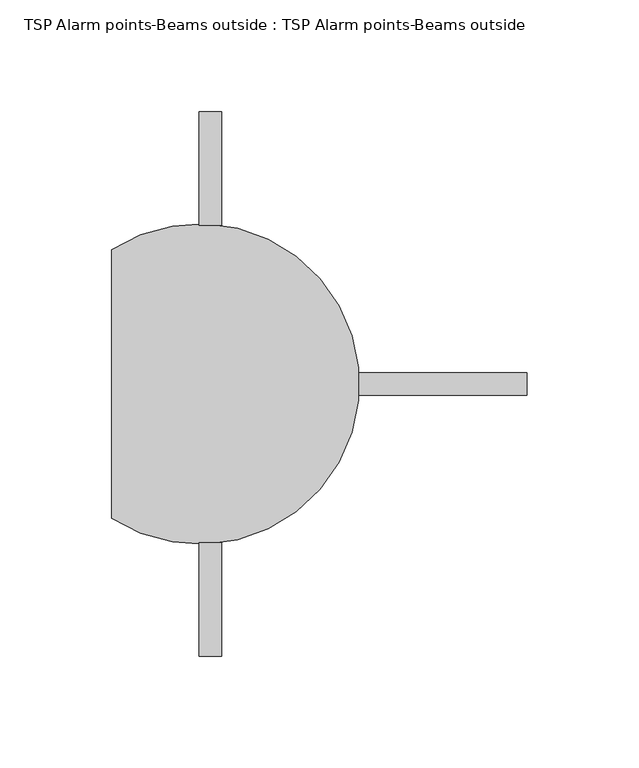
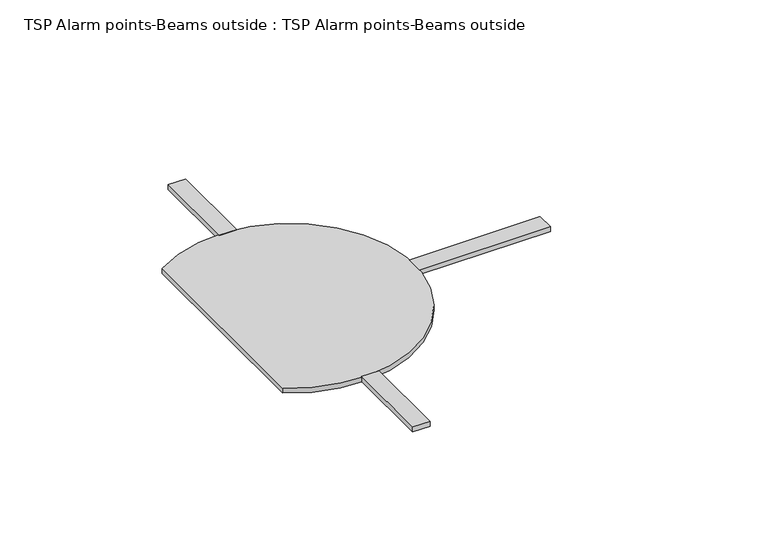
"""IFC4 building model written with IfcOpenShell, lengths in millimetres: proxy geometry, TSP Alarm points-Beams outside : TSP Alarm points-Beams outside."""

from ifc_helpers import new_model, si_unit, point, frame_2d, origin, origin_with_axes, place, context, project, spatial, polyline, circle_curve, trimmed, segment, composite_curve, outline, extrude, source, transform, mapped, element, save


def tsp_alarm_points_beams_outside_tsp_alarm_points_beams_36a8186e(model_context):
    return source(origin(), model_context, "Body", "SweptSolid", [
        extrude(outline(polyline([(75.7016567, 5.0), (75.7016567, -5.0), (0.5268886, -5.0), (0.5268886, 5.0), (75.7016567, 5.0)])), origin_with_axes(), (0.0, 0.0, 1.0), 3.0),
        extrude(outline(polyline([(-70.9090909, 121.6107476), (-60.9090909, 121.6107476), (-60.9090909, 70.9090909), (-70.9090909, 70.9090909), (-70.9090909, 121.6107476)])), origin_with_axes(), (0.0, 0.0, 1.0), 3.0),
        extrude(outline(polyline([(-70.9090909, -121.6107476), (-70.9090909, -70.9090909), (-60.9090909, -70.9090909), (-60.9090909, -121.6107476), (-70.9090909, -121.6107476)])), origin_with_axes(), (0.0, 0.0, 1.0), 3.0),
        extrude(outline(composite_curve([segment(trimmed(circle_curve(frame_2d((-70.9090909, 0.0)), 71.6107476), [point((-110.0, 60.0))], [point((-110.0, -60.0))], False, "CARTESIAN"), True, "CONTINUOUS"), segment(polyline([(-110.0, -60.0), (-110.0, 60.0)]), True, "CONTINUOUS")], self_intersect=False)), origin_with_axes(), (0.0, 0.0, 1.0), 3.0),
    ])


if __name__ == "__main__":
    model = new_model("IFC4")
    model_context = context("Model", 3, world=origin())
    ifc_project = project(units=[si_unit("LENGTHUNIT", "METRE", prefix="MILLI")], contexts=[model_context])
    site = spatial("IfcSite", under=ifc_project)
    building = spatial("IfcBuilding", under=site)
    placement = place(None, origin())
    tsp_alarm_points_beams_outside_tsp_alarm_points_beams_shape = tsp_alarm_points_beams_outside_tsp_alarm_points_beams_36a8186e(model_context)
    element("IfcBuildingElementProxy", 1, Name="TSP Alarm points-Beams outside : TSP Alarm points-Beams outside", ObjectType="TSP Alarm points-Beams outside : TSP Alarm points-Beams outside", at=placement, inside=building, context=model_context, shape_type="MappedRepresentation", body=[
        mapped(tsp_alarm_points_beams_outside_tsp_alarm_points_beams_shape, transform((0.0, 0.0, 0.0), x_axis=(1.0, 0.0, 0.0), y_axis=(0.0, 1.0, 0.0), z_axis=(0.0, 0.0, 1.0))),
    ])
    save(model, "model.ifc")

# Revit data of these elements
# Type "TSP Alarm points-Beams outside : TSP Alarm points-Beams outside"
#   Model = "TSP_ELECABO"
#   Default Elevation = 0
# Element 1 (IfcBuildingElementProxy, "TSP Alarm points-Beams outside : TSP Alarm points-Beams outside")
#   Materials on its faces: "Aluminum, Anodized Blue", "Plastic, Opaque Black"
# Materials
#   "Aluminum, Anodized Blue": class "Metal", colour RGB 120 120 120, transparency 0, Description = "Anodized aluminum, blue", Cost = 0
#   "Plastic, Opaque Black": class "Plastic", colour RGB 0 0 0, transparency 0.7, Description = "Plastic, generic, opaque black", Cost = 0
